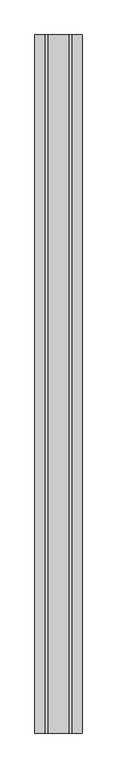
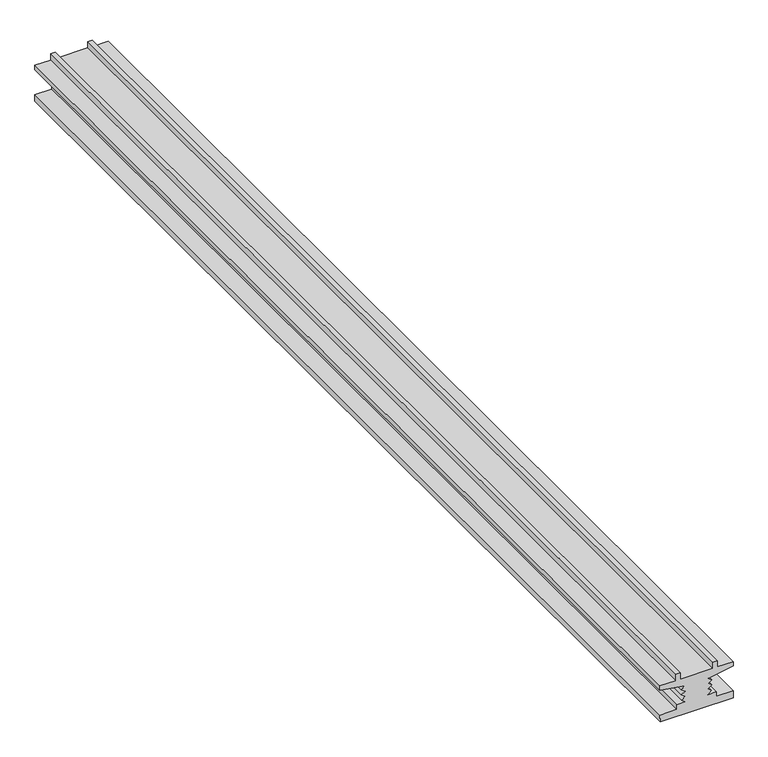
"""IFC4 building model written with IfcOpenShell, lengths in millimetres: proxy geometry, Bison pedestal003 : Bison pedestal003."""

from ifc_helpers import new_model, si_unit, frame, origin, place, context, project, spatial, polyline, outline, extrude, source, transform, mapped, element, save


def generic_models_3fa60072(model_context):
    return source(origin(), model_context, "Body", "SweptSolid", [
        extrude(outline(polyline([(36437.1701104, -5885.2048082), (36450.5703125, -5885.0756836), (36450.5703125, -5915.9145508), (36459.5256875, -5915.9145508), (36459.5256875, -5932.0966797), (36465.4085, -5925.0351562), (36470.5608437, -5931.6552734), (36476.00225, -5924.5942383), (36481.1506875, -5931.3613281), (36486.2170937, -5924.2119141), (36491.3108437, -5930.6450195), (36499.0842812, -5885.0756836), (36507.392875, -5885.0756836), (36507.392875, -5914.5620117), (36519.7249062, -5914.5620117), (36519.7249062, -5922.3354492), (36507.392875, -5922.3354492), (36507.392875, -5982.9155273), (36519.7249062, -5982.9155273), (36519.7249062, -5990.6889648), (36507.392875, -5990.6889648), (36507.392875, -6020.175293), (36499.0842812, -6020.175293), (36491.3108437, -5974.605957), (36486.2170937, -5981.0390625), (36481.1506875, -5973.8896484), (36476.00225, -5980.6567383), (36470.5608437, -5973.5957031), (36465.4085, -5980.2158203), (36459.5256875, -5973.1542969), (36459.5256875, -5989.3364258), (36450.5703125, -5989.3364258), (36450.5703125, -6020.175293), (36437.1701104, -6020.0461683), (36437.1701104, -5952.6254883), (36437.1701104, -5885.2048082)])), frame((0.0, -1052.8906574, 0.0), z_axis=(0.0, 1.0, 0.0), x_axis=(0.0, 0.0, 1.0)), (0.0, 0.0, 1.0), 2000.0),
    ])


if __name__ == "__main__":
    model = new_model("IFC4")
    model_context = context("Model", 3, world=origin())
    ifc_project = project(units=[si_unit("LENGTHUNIT", "METRE", prefix="MILLI")], contexts=[model_context])
    site = spatial("IfcSite", under=ifc_project)
    building = spatial("IfcBuilding", under=site)
    placement = place(None, origin())
    generic_models_shape = generic_models_3fa60072(model_context)
    element("IfcBuildingElementProxy", 1, Name="Bison pedestal003 : Bison pedestal003", ObjectType="Bison pedestal003 : Bison pedestal003", at=placement, inside=building, context=model_context, shape_type="MappedRepresentation", body=[
        mapped(generic_models_shape, transform((0.0, 0.0, 0.0), x_axis=(1.0, 0.0, 0.0), y_axis=(0.0, 1.0, 0.0), z_axis=(0.0, 0.0, 1.0))),
    ])
    save(model, "model.ifc")

# Revit data of these elements
# Type "Bison pedestal003 : Bison pedestal003"
#   NameOverride = "Bison pedestal003"
# Element 1 (IfcBuildingElementProxy, "Bison pedestal003 : Bison pedestal003")
#   Materials on its faces: "BUZON PEDESTAL"
# Materials
#   "BUZON PEDESTAL": class "Unassigned", colour RGB 66 66 66, transparency 0
